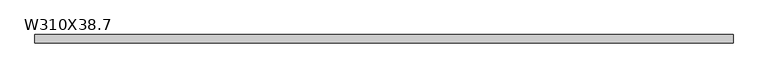
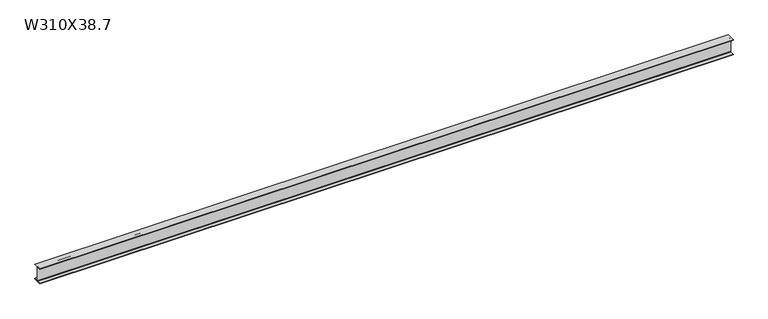
"""IFC4 building model written with IfcOpenShell, lengths in millimetres: beam geometry, M_W Shapes : W310X38.7."""

from ifc_helpers import new_model, si_unit, point, frame, frame_2d, origin, place, context, project, spatial, polyline, circle_curve, trimmed, segment, composite_curve, outline, extrude, source, transform, mapped, element, save


def w310x38_7_298f7b34(model_context):
    return source(origin(), model_context, "Body", "SweptSolid", [
        extrude(outline(composite_curve([segment(polyline([(82.5, -145.35), (82.5, -155.0), (-82.5, -155.0), (-82.5, -145.35), (-10.57, -145.35)]), True, "CONTINUOUS"), segment(trimmed(circle_curve(frame_2d((-10.57, -137.7)), 7.65), [point((-10.57, -145.35))], [point((-2.92, -137.7))], True, "CARTESIAN"), True, "CONTINUOUS"), segment(polyline([(-2.92, -137.7), (-2.92, 137.7)]), True, "CONTINUOUS"), segment(trimmed(circle_curve(frame_2d((-10.57, 137.7)), 7.65), [point((-2.92, 137.7))], [point((-10.57, 145.35))], True, "CARTESIAN"), True, "CONTINUOUS"), segment(polyline([(-10.57, 145.35), (-82.5, 145.35), (-82.5, 155.0), (82.5, 155.0), (82.5, 145.35), (10.57, 145.35)]), True, "CONTINUOUS"), segment(trimmed(circle_curve(frame_2d((10.57, 137.7)), 7.65), [point((10.57, 145.35))], [point((2.92, 137.7))], True, "CARTESIAN"), True, "CONTINUOUS"), segment(polyline([(2.92, 137.7), (2.92, -137.7)]), True, "CONTINUOUS"), segment(trimmed(circle_curve(frame_2d((10.57, -137.7)), 7.65), [point((2.92, -137.7))], [point((10.57, -145.35))], True, "CARTESIAN"), True, "CONTINUOUS"), segment(polyline([(10.57, -145.35), (82.5, -145.35)]), True, "CONTINUOUS")], self_intersect=False)), frame((-6666.25, 0.0, 0.0), z_axis=(1.0, 0.0, 0.0), x_axis=(0.0, 1.0, 0.0)), (0.0, 0.0, 1.0), 13656.7),
    ])


if __name__ == "__main__":
    model = new_model("IFC4")
    model_context = context("Model", 3, world=origin())
    ifc_project = project(units=[si_unit("LENGTHUNIT", "METRE", prefix="MILLI")], contexts=[model_context])
    site = spatial("IfcSite", under=ifc_project)
    building = spatial("IfcBuilding", under=site)
    placement = place(None, origin())
    w310x38_7_shape = w310x38_7_298f7b34(model_context)
    element("IfcBeam", 1, ObjectType="M_W Shapes : W310X38.7", at=placement, inside=building, context=model_context, shape_type="MappedRepresentation", body=[
        mapped(w310x38_7_shape, transform((0.0, 0.0, 0.0), x_axis=(1.0, 0.0, 0.0), y_axis=(0.0, 1.0, 0.0), z_axis=(0.0, 0.0, 1.0))),
    ])
    save(model, "model.ifc")

# Revit data of these elements
# Type "M_W Shapes : W310X38.7"
#   Section Name Key = "W12x26"
#   Width = 165 mm
#   Web Thickness = 5.84 mm
#   Web Fillet = 7.65 mm
#   Warping Constant = 163000 cm⁶
#   Torsional Moment of Inertia = 12.5 cm⁴
#   Section Area = 49.4 cm²
#   Plastic Modulus weak axis = 0.00473217 (stored number, unit not read)
#   Plastic Modulus strong axis = 0.0215419 (stored number, unit not read)
#   Perimeter = 1.25 m²/m
#   Nominal Weight = 379.516 N/m
#   Moment of Inertia weak axis = 720 cm⁴
#   Moment of Inertia strong axis = 8490 cm⁴
#   Height = 310 mm
#   Flange Thickness = 9.65 mm
#   Elastic Modulus weak axis = 0.00309003 (stored number, unit not read)
#   Elastic Modulus strong axis = 0.0193171 (stored number, unit not read)
#   Centroid Vertical = 155 mm
#   Centroid Horizontal = 82.5 mm
#   Length [instance default] = 1.5 m
#   Structural Material [instance default] = Steel, 45-345
#   Assembly Code = ""
# Element 1 (IfcBeam, "M_W Shapes : W310X38.7")
#   Materials on its faces: "Steel, 45-345"
# Materials
#   "Steel, 45-345": class "Metal", colour RGB 189 187 185, transparency 0, Description = "Steel 345 MPa", Cost = 0
